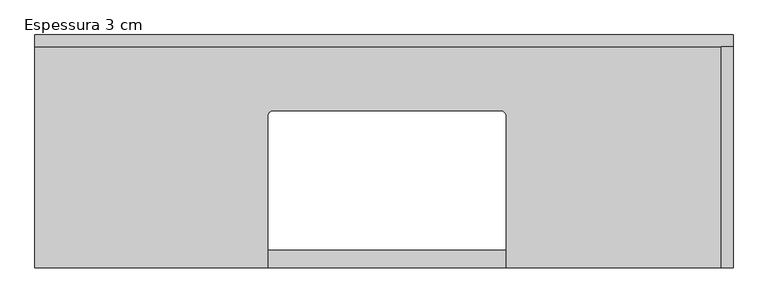
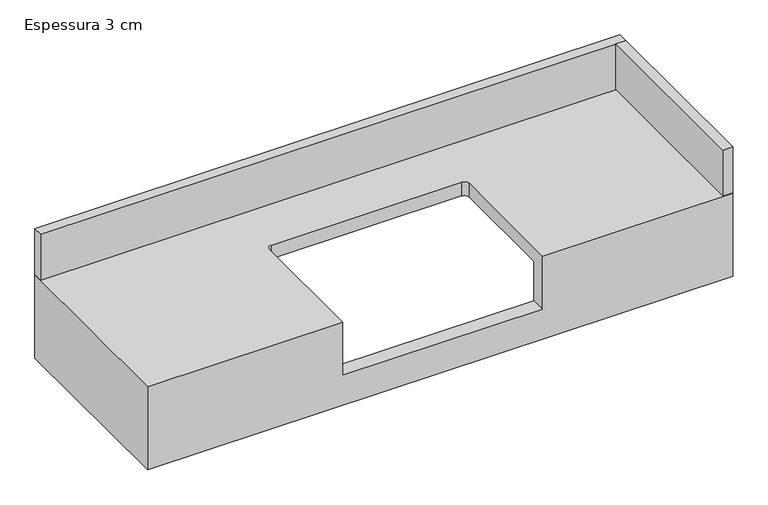
"""IFC4 building model written with IfcOpenShell, lengths in millimetres: furniture geometry, CC_BANCADA BANHEIRO COM CUBA_CANTO RETO : Espessura 3 cm."""

from ifc_helpers import new_model, si_unit, frame, origin, place, context, project, spatial, polyline, circle_curve, outline, extrude, source, transform, mapped, element, save
from ifc_brep_helpers import plane_surface, revolved_surface, advanced_brep


def espessura_3_cm_493110b7(model_context):
    return source(origin(), model_context, "Body", "SolidModel", [
        advanced_brep(
        [(750.0, 300.0, 860.0), (-450.0, 300.0, 860.0), (-450.0, -100.0, 860.0), (-50.0, -100.0, 860.0), (-50.0, 160.0, 860.0), (-40.0, 170.0, 860.0), (350.0, 170.0, 860.0), (360.0, 160.0, 860.0), (360.0, -100.0, 860.0), (750.0, -100.0, 860.0), (750.0, 300.0, 680.0), (720.0, 300.0, 680.0), (720.0, 300.0, 830.0), (-420.0, 300.0, 830.0), (-420.0, 300.0, 680.0), (-450.0, 300.0, 680.0), (-450.0, -100.0, 680.0), (750.0, -100.0, 680.0), (360.0, -100.0, 745.0), (-50.0, -100.0, 745.0), (720.0, -70.0, 830.0), (360.0, -70.0, 830.0), (360.0, 160.0, 830.0), (350.0, 170.0, 830.0), (-40.0, 170.0, 830.0), (-50.0, 160.0, 830.0), (-50.0, -70.0, 830.0), (-420.0, -70.0, 830.0), (-420.0, -70.0, 680.0), (-50.0, -70.0, 745.0), (360.0, -70.0, 745.0), (720.0, -70.0, 680.0)],
        [
            (0, 1),
            (1, 2),
            (2, 3),
            (3, 4),
            (4, 5, circle_curve(frame((-40.0, 160.0, 860.0), z_axis=(0.0, 0.0, -1.0), x_axis=(0.0, 1.0, 0.0)), 10.0)),
            (5, 6),
            (6, 7, circle_curve(frame((350.0, 160.0, 860.0), z_axis=(0.0, 0.0, -1.0), x_axis=(0.0, 1.0, 0.0)), 10.0)),
            (7, 8),
            (8, 9),
            (9, 0),
            (0, 10),
            (10, 11),
            (11, 12),
            (12, 13),
            (13, 14),
            (14, 15),
            (15, 1),
            (15, 16),
            (16, 2),
            (16, 17),
            (17, 9),
            (8, 18),
            (18, 19),
            (19, 3),
            (17, 10),
            (12, 20),
            (20, 21),
            (21, 22),
            (22, 23, circle_curve(frame((350.0, 160.0, 830.0), z_axis=(0.0, 0.0, 1.0), x_axis=(0.0, 1.0, 0.0)), 10.0)),
            (23, 24),
            (24, 25, circle_curve(frame((-40.0, 160.0, 830.0), z_axis=(0.0, 0.0, 1.0), x_axis=(0.0, 1.0, 0.0)), 10.0)),
            (25, 26),
            (26, 27),
            (27, 13),
            (27, 28),
            (28, 14),
            (26, 29),
            (29, 30),
            (30, 21),
            (20, 31),
            (31, 28),
            (11, 31),
            (5, 24),
            (23, 6),
            (18, 30),
            (29, 19),
            (4, 25),
            (7, 22),
        ],
        [
            plane_surface(frame((-450.0, 300.0, 860.0), z_axis=(0.0, 0.0, 1.0), x_axis=(-1.0, 0.0, 0.0))),
            plane_surface(frame((750.0, 300.0, 860.0), z_axis=(0.0, 1.0, 0.0), x_axis=(0.0, 0.0, -1.0))),
            plane_surface(frame((-450.0, 300.0, 860.0), z_axis=(-1.0, 0.0, 0.0), x_axis=(0.0, 0.0, -1.0))),
            plane_surface(frame((-450.0, -100.0, 860.0), z_axis=(0.0, -1.0, 0.0), x_axis=(0.0, 0.0, -1.0))),
            plane_surface(frame((750.0, -100.0, 860.0), z_axis=(1.0, 0.0, 0.0), x_axis=(0.0, 0.0, -1.0))),
            plane_surface(frame((-420.0, 300.0, 830.0), z_axis=(0.0, 0.0, -1.0), x_axis=(-1.0, 0.0, 0.0))),
            plane_surface(frame((-420.0, 300.0, 830.0), z_axis=(1.0, 0.0, 0.0), x_axis=(0.0, 0.0, -1.0))),
            plane_surface(frame((-420.0, -70.0, 830.0), z_axis=(0.0, 1.0, 0.0), x_axis=(0.0, 0.0, -1.0))),
            plane_surface(frame((720.0, -70.0, 830.0), z_axis=(-1.0, 0.0, 0.0), x_axis=(0.0, 0.0, -1.0))),
            plane_surface(frame((750.0, -100.0, 680.0), z_axis=(0.0, 0.0, -1.0), x_axis=(0.0, 1.0, 0.0))),
            plane_surface(frame((-40.0, 170.0, 745.0), z_axis=(0.0, -1.0, 0.0), x_axis=(0.0, 0.0, 1.0))),
            plane_surface(frame((350.0, 170.0, 745.0), z_axis=(0.0, 0.0, 1.0), x_axis=(1.0, 0.0, 0.0))),
            revolved_surface(polyline([(-40.0, 170.0, 830.0), (-40.0, 170.0, 860.0)]), (-40.0, 160.0, 900.0), (0.0, 0.0, -1.0)),
            plane_surface(frame((-50.0, -230.0, 745.0), z_axis=(1.0, 0.0, 0.0), x_axis=(0.0, 0.0, 1.0))),
            plane_surface(frame((360.0, 160.0, 745.0), z_axis=(-1.0, 0.0, 0.0), x_axis=(0.0, 0.0, 1.0))),
            revolved_surface(polyline([(350.0, 170.0, 830.0), (350.0, 170.0, 860.0)]), (350.0, 160.0, 900.0), (0.0, 0.0, -1.0)),
        ],
        [
            (0, [[1, 2, 3, 4, 5, 6, 7, 8, 9, 10]]),
            (1, [[-1, 11, 12, 13, 14, 15, 16, 17]]),
            (2, [[-2, -17, 18, 19]]),
            (3, [[-3, -19, 20, 21, -9, 22, 23, 24]]),
            (4, [[-10, -21, 25, -11]]),
            (5, [[26, 27, 28, 29, 30, 31, 32, 33, 34, -14]]),
            (6, [[-34, 35, 36, -15]]),
            (7, [[-33, 37, 38, 39, -27, 40, 41, -35]]),
            (8, [[-26, -13, 42, -40]]),
            (9, [[-12, -25, -20, -18, -16, -36, -41, -42]]),
            (10, [[-6, 43, -30, 44]]),
            (11, [[-23, 45, -38, 46]]),
            (12, [[-5, 47, -31, -43]]),
            (13, [[-4, -24, -46, -37, -32, -47]]),
            (14, [[-8, 48, -28, -39, -45, -22]]),
            (15, [[-7, -44, -29, -48]]),
        ],
    ),
        extrude(outline(polyline([(730.0, 280.0), (750.0, 280.0), (750.0, -100.0), (730.0, -100.0), (730.0, 280.0)])), frame((0.0, 0.0, 860.0), z_axis=(0.0, 0.0, 1.0), x_axis=(1.0, 0.0, 0.0)), (0.0, 0.0, 1.0), 100.0),
        extrude(outline(polyline([(750.0, 300.0), (750.0, 280.0), (-450.0, 280.0), (-450.0, 300.0), (750.0, 300.0)])), frame((0.0, 0.0, 860.0), z_axis=(0.0, 0.0, 1.0), x_axis=(1.0, 0.0, 0.0)), (0.0, 0.0, 1.0), 100.0),
    ])


if __name__ == "__main__":
    model = new_model("IFC4")
    model_context = context("Model", 3, world=origin())
    ifc_project = project(units=[si_unit("LENGTHUNIT", "METRE", prefix="MILLI")], contexts=[model_context])
    site = spatial("IfcSite", under=ifc_project)
    building = spatial("IfcBuilding", under=site)
    placement = place(None, origin())
    espessura_3_cm_shape = espessura_3_cm_493110b7(model_context)
    element("IfcFurniture", 1, ObjectType="CC_BANCADA BANHEIRO COM CUBA_CANTO RETO : Espessura 3 cm", at=placement, inside=building, context=model_context, shape_type="MappedRepresentation", body=[
        mapped(espessura_3_cm_shape, transform((0.0, 0.0, 0.0), x_axis=(1.0, 0.0, 0.0), y_axis=(0.0, 1.0, 0.0), z_axis=(0.0, 0.0, 1.0))),
    ])
    save(model, "model.ifc")

# Revit data of these elements
# Type "CC_BANCADA BANHEIRO COM CUBA_CANTO RETO : Espessura 3 cm"
#   Uso HS [instance default] = ""
#   h TESTEIRA AUX [instance default] = 0.15 m
#   Altura testeira [instance default] = 0.15 m
#   Altura rodapia [instance default] = 0.10 m
#   Espessura rodapia [instance default] = 0.02 m
#   Prof/2 [instance default] = 0.20 m
#   Offset cuba esquerda [instance default] = 0.40 m
#   Depth [instance default] = 1.20 m
#   Width [instance default] = 0.40 m
#   Espessura bancada = 0.03 m
#   Comprimento [instance default] = 1.20 m
#   Height [instance default] = 0.86 m
#   Testeira [instance default] = yes
#   Rodapia fundo [instance default] = no
#   Rodapia esquerda [instance default] = no
#   Rodapia direita [instance default] = no
#   Material porta-toalha [instance default] = .CROMADO
#   Material hidráulico [instance default] = .CROMADO
#   Material cuba [instance default] = .PORCELANA BRANCA
#   Material bancada [instance default] = .GRANITO_BRANCO_ITAUNAS
#   Assembly Code = ""
# Element 1 (IfcFurniture, "CC_BANCADA BANHEIRO COM CUBA_CANTO RETO : Espessura 3 cm")
#   Uso HS = "BANHO SUÍTE 1"
#   Rodapia fundo = yes
#   Rodapia direita = yes
#   Materials on its faces: ".GRANITO_BRANCO_ITAUNAS"
# Materials
#   ".CROMADO": class "CC_METAIS", colour RGB 211 223 226, transparency 0, Cost = 0
#   ".PORCELANA BRANCA": class "CC_PORCELANA", colour RGB 230 230 230, transparency 0, Cost = 0
#   ".GRANITO_BRANCO_ITAUNAS": class ".CC_PEDRA REVEST.", colour RGB 202 195 174, transparency 0, Description = "Revestimento em granito", Cost = 0
